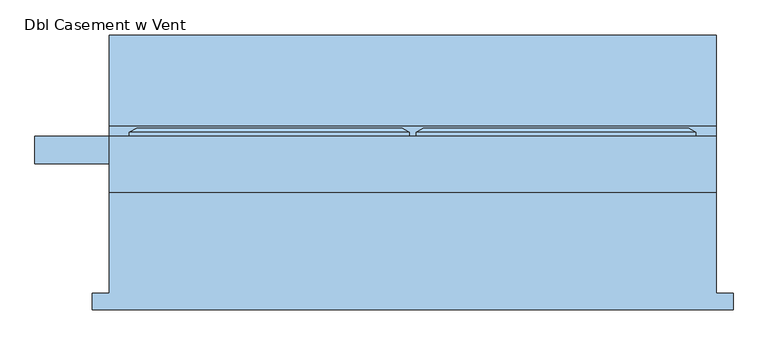
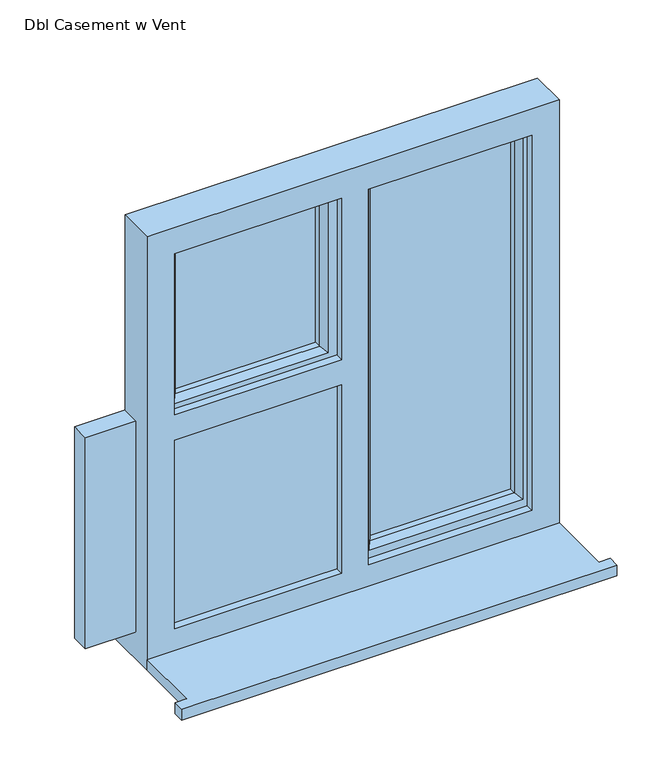
"""IFC4 building model written with IfcOpenShell, lengths in millimetres: window geometry, Dbl Casement w Vent : Doublel Casement with Vent 900w x 1000h."""

from ifc_helpers import new_model, si_unit, frame, origin, place, context, project, spatial, polyline, outline, extrude, faceted_brep, source, transform, mapped, element, save


def dbl_casement_w_vent_ca28e73d(model_context):
    return source(origin(), model_context, "Body", "SolidModel", [
        extrude(outline(polyline([(-760.0, -182.7934322), (-760.0, -157.7934322), (-735.0, -157.7934322), (-735.0, -8.2934322), (165.0, -8.2934322), (165.0, -157.7934322), (190.0, -157.7934322), (190.0, -182.7934322), (-760.0, -182.7934322)])), frame((0.0, 0.0, 1110.0), z_axis=(0.0, 0.0, 1.0), x_axis=(1.0, 0.0, 0.0)), (0.0, 0.0, 1.0), 25.0),
        faceted_brep([(-705.0, 74.7065678, 2080.0), (-705.0, 80.4800705, 2080.0), (-705.0, 80.4800705, 1650.0), (-705.0, 74.7065678, 1650.0), (-695.0, 9.7065678, 2070.0), (-695.0, 74.7065678, 2070.0), (-695.0, 74.7065678, 1660.0), (-695.0, 9.7065678, 1660.0), (-655.0, 24.1994677, 2030.0), (-665.1480377, 9.7065678, 2040.1480377), (-665.1480377, 9.7065678, 1689.8519623), (-655.0, 24.1994677, 1700.0), (-655.0, 38.7065678, 2030.0), (-655.0, 38.7065678, 1700.0), (-665.0, 62.7065678, 2040.0), (-665.0, 38.7065678, 2040.0), (-665.0, 38.7065678, 1690.0), (-665.0, 62.7065678, 1690.0), (-655.0, 80.4800705, 2030.0), (-655.0, 62.7065678, 2030.0), (-655.0, 62.7065678, 1700.0), (-655.0, 80.4800705, 1700.0), (-672.4457548, 86.2535732, 2047.4457548), (-672.4457548, 86.2535732, 1682.5542452), (-694.2153903, 86.2535732, 2069.2153903), (-694.2153903, 86.2535732, 1660.7846097), (-290.0, 80.4800705, 1650.0), (-290.0, 74.7065678, 1650.0), (-300.0, 74.7065678, 1660.0), (-300.0, 9.7065678, 1660.0), (-329.8519623, 9.7065678, 1689.8519623), (-340.0, 24.1994677, 1700.0), (-340.0, 38.7065678, 1700.0), (-330.0, 38.7065678, 1690.0), (-330.0, 62.7065678, 1690.0), (-340.0, 62.7065678, 1700.0), (-340.0, 80.4800705, 1700.0), (-322.5542452, 86.2535732, 1682.5542452), (-300.7846097, 86.2535732, 1660.7846097), (-290.0, 80.4800705, 2080.0), (-290.0, 74.7065678, 2080.0), (-300.0, 74.7065678, 2070.0), (-300.0, 9.7065678, 2070.0), (-329.8519623, 9.7065678, 2040.1480377), (-340.0, 24.1994677, 2030.0), (-340.0, 38.7065678, 2030.0), (-330.0, 38.7065678, 2040.0), (-330.0, 62.7065678, 2040.0), (-340.0, 62.7065678, 2030.0), (-340.0, 80.4800705, 2030.0), (-322.5542452, 86.2535732, 2047.4457548), (-300.7846097, 86.2535732, 2069.2153903)], [[[0, 1, 2, 3]], [[4, 5, 6, 7]], [[8, 9, 10, 11]], [[12, 8, 11, 13]], [[14, 15, 16, 17]], [[18, 19, 20, 21]], [[22, 18, 21, 23]], [[1, 24, 25, 2]], [[3, 2, 26, 27]], [[7, 6, 28, 29]], [[11, 10, 30, 31]], [[13, 11, 31, 32]], [[17, 16, 33, 34]], [[21, 20, 35, 36]], [[23, 21, 36, 37]], [[2, 25, 38, 26]], [[27, 26, 39, 40]], [[29, 28, 41, 42]], [[31, 30, 43, 44]], [[32, 31, 44, 45]], [[34, 33, 46, 47]], [[36, 35, 48, 49]], [[37, 36, 49, 50]], [[26, 38, 51, 39]], [[40, 39, 1, 0]], [[3, 27, 40, 0], [5, 41, 28, 6]], [[42, 41, 5, 4]], [[7, 29, 42, 4], [9, 43, 30, 10]], [[44, 43, 9, 8]], [[45, 44, 8, 12]], [[15, 46, 33, 16], [13, 32, 45, 12]], [[47, 46, 15, 14]], [[17, 34, 47, 14], [19, 48, 35, 20]], [[49, 48, 19, 18]], [[50, 49, 18, 22]], [[24, 51, 38, 25], [23, 37, 50, 22]], [[39, 51, 24, 1]]]),
        extrude(outline(polyline([(95.0, 38.7065678), (-240.0, 38.7065678), (-240.0, 62.7065678), (95.0, 62.7065678), (95.0, 38.7065678)])), frame((0.0, 0.0, 1203.0), z_axis=(0.0, 0.0, 1.0), x_axis=(1.0, 0.0, 0.0)), (0.0, 0.0, 1.0), 837.0),
        extrude(outline(polyline([(-330.0, 38.7065678), (-665.0, 38.7065678), (-665.0, 62.7065678), (-330.0, 62.7065678), (-330.0, 38.7065678)])), frame((0.0, 0.0, 1690.0), z_axis=(0.0, 0.0, 1.0), x_axis=(1.0, 0.0, 0.0)), (0.0, 0.0, 1.0), 350.0),
        extrude(outline(polyline([(-695.0, 33.7065678), (-300.0, 33.7065678), (-300.0, 9.7065678), (-695.0, 9.7065678), (-695.0, 33.7065678)])), frame((0.0, 0.0, 1173.0), z_axis=(0.0, 0.0, 1.0), x_axis=(1.0, 0.0, 0.0)), (0.0, 0.0, 1.0), 457.0),
        faceted_brep([(165.0, -8.2934322, 2110.0), (-735.0, -8.2934322, 2110.0), (-735.0, -8.2934322, 1110.0), (165.0, -8.2934322, 1110.0), (-675.0, -8.2934322, 1185.0), (-675.0, -8.2934322, 1620.0), (-310.0, -8.2934322, 1620.0), (-310.0, -8.2934322, 1185.0), (-675.0, -8.2934322, 2050.0), (-310.0, -8.2934322, 2050.0), (-310.0, -8.2934322, 1678.0), (-675.0, -8.2934322, 1678.0), (-252.0, -8.2934322, 2050.0), (105.0, -8.2934322, 2050.0), (105.0, -8.2934322, 1185.0), (-252.0, -8.2934322, 1185.0), (-735.0, 74.7065678, 2110.0), (-735.0, 74.7065678, 1161.0), (-735.0, 89.7065678, 1159.68767), (-735.0, 89.7065678, 1154.7449676), (-735.0, 224.7065678, 1143.8088847), (-735.0, 224.7065678, 1110.0), (165.0, 74.7065678, 2110.0), (165.0, 74.7065678, 1161.0), (-310.0, 74.7065678, 1173.0), (-310.0, 74.7065678, 1620.0), (-695.0, 74.7065678, 1620.0), (-695.0, 74.7065678, 1173.0), (-310.0, 74.7065678, 2070.0), (-695.0, 74.7065678, 2070.0), (-695.0, 74.7065678, 1660.0), (-310.0, 74.7065678, 1660.0), (125.0, 74.7065678, 1173.0), (125.0, 74.7065678, 2070.0), (-270.0, 74.7065678, 2070.0), (-270.0, 74.7065678, 1173.0), (-695.0, 9.7065678, 2070.0), (-695.0, 9.7065678, 1660.0), (-695.0, 9.7065678, 1630.0), (-695.0, 9.7065678, 1173.0), (-695.0, 33.7065678, 1620.0), (-695.0, 33.7065678, 1630.0), (-300.0, 9.7065678, 2070.0), (-300.0, 9.7065678, 1660.0), (-310.0, 9.7065678, 2050.0), (-675.0, 9.7065678, 2050.0), (-675.0, 9.7065678, 1678.0), (-310.0, 9.7065678, 1678.0), (-270.0, 9.7065678, 2070.0), (125.0, 9.7065678, 2070.0), (125.0, 9.7065678, 1173.0), (-270.0, 9.7065678, 1173.0), (105.0, 9.7065678, 2050.0), (-252.0, 9.7065678, 2050.0), (-252.0, 9.7065678, 1185.0), (105.0, 9.7065678, 1185.0), (-300.0, 9.7065678, 1173.0), (-300.0, 9.7065678, 1630.0), (-675.0, 9.7065678, 1185.0), (-310.0, 9.7065678, 1185.0), (-310.0, 9.7065678, 1620.0), (-675.0, 9.7065678, 1620.0), (-310.0, 33.7065678, 2070.0), (-300.0, 33.7065678, 2070.0), (165.0, 224.7065678, 1110.0), (165.0, 224.7065678, 1143.8088847), (165.0, 89.7065678, 1154.7449676), (165.0, 89.7065678, 1159.68767), (-300.0, 33.7065678, 1660.0), (-300.0, 33.7065678, 1630.0), (-300.0, 33.7065678, 1173.0), (-310.0, 33.7065678, 1660.0), (-310.0, 33.7065678, 1173.0), (-310.0, 33.7065678, 1620.0)], [[[0, 1, 2, 3], [4, 5, 6, 7], [8, 9, 10, 11], [12, 13, 14, 15]], [[1, 16, 17, 18, 19, 20, 21, 2]], [[16, 22, 23, 17], [24, 25, 26, 27], [28, 29, 30, 31], [32, 33, 34, 35]], [[29, 36, 37, 30]], [[38, 39, 27, 26, 40, 41]], [[36, 42, 43, 37], [44, 45, 46, 47]], [[48, 49, 50, 51], [52, 53, 54, 55]], [[56, 39, 38, 57], [58, 59, 60, 61]], [[45, 8, 11, 46]], [[4, 58, 61, 5]], [[1, 0, 22, 16]], [[36, 29, 28, 62, 63, 42]], [[33, 49, 48, 34]], [[8, 45, 44, 9]], [[52, 13, 12, 53]], [[22, 0, 3, 64, 65, 66, 67, 23]], [[33, 32, 50, 49]], [[13, 52, 55, 14]], [[43, 42, 63, 68]], [[69, 70, 56, 57]], [[63, 62, 71, 68]], [[72, 70, 69, 41, 40, 73]], [[62, 28, 31, 71]], [[24, 72, 73, 25]], [[35, 34, 48, 51]], [[53, 12, 15, 54]], [[9, 44, 47, 10]], [[59, 7, 6, 60]], [[64, 3, 2, 21]], [[65, 64, 21, 20]], [[66, 65, 20, 19]], [[67, 66, 19, 18]], [[23, 67, 18, 17]], [[24, 27, 39, 56, 70, 72]], [[32, 35, 51, 50]], [[15, 14, 55, 54]], [[59, 58, 4, 7]], [[57, 38, 41, 69]], [[26, 25, 73, 40]], [[31, 30, 37, 43, 68, 71]], [[47, 46, 11, 10]], [[61, 60, 6, 5]]]),
        extrude(outline(polyline([(1660.0, -675.0), (1660.0, -845.0), (1173.0, -845.0), (1173.0, -310.0), (1343.0, -310.0), (1343.0, -675.0), (1660.0, -675.0)])), frame((0.0, 33.7065678, 0.0), z_axis=(0.0, 1.0, 0.0), x_axis=(0.0, 0.0, 1.0)), (0.0, 0.0, 1.0), 41.0),
        faceted_brep([(-280.0, 74.7065678, 2080.0), (-280.0, 80.4800705, 2080.0), (-280.0, 80.4800705, 1163.0), (-280.0, 74.7065678, 1163.0), (-270.0, 9.7065678, 2070.0), (-270.0, 74.7065678, 2070.0), (-270.0, 74.7065678, 1173.0), (-270.0, 9.7065678, 1173.0), (-230.0, 24.1994677, 2030.0), (-240.1480377, 9.7065678, 2040.1480377), (-240.1480377, 9.7065678, 1202.8519623), (-230.0, 24.1994677, 1213.0), (-230.0, 38.7065678, 2030.0), (-230.0, 38.7065678, 1213.0), (-240.0, 62.7065678, 2040.0), (-240.0, 38.7065678, 2040.0), (-240.0, 38.7065678, 1203.0), (-240.0, 62.7065678, 1203.0), (-230.0, 80.4800705, 2030.0), (-230.0, 62.7065678, 2030.0), (-230.0, 62.7065678, 1213.0), (-230.0, 80.4800705, 1213.0), (-247.4457548, 86.2535732, 2047.4457548), (-247.4457548, 86.2535732, 1195.5542452), (-269.2153903, 86.2535732, 2069.2153903), (-269.2153903, 86.2535732, 1173.7846097), (135.0, 80.4800705, 1163.0), (135.0, 74.7065678, 1163.0), (125.0, 74.7065678, 1173.0), (125.0, 9.7065678, 1173.0), (95.1480377, 9.7065678, 1202.8519623), (85.0, 24.1994677, 1213.0), (85.0, 38.7065678, 1213.0), (95.0, 38.7065678, 1203.0), (95.0, 62.7065678, 1203.0), (85.0, 62.7065678, 1213.0), (85.0, 80.4800705, 1213.0), (102.4457548, 86.2535732, 1195.5542452), (124.2153903, 86.2535732, 1173.7846097), (135.0, 80.4800705, 2080.0), (135.0, 74.7065678, 2080.0), (125.0, 74.7065678, 2070.0), (125.0, 9.7065678, 2070.0), (95.1480377, 9.7065678, 2040.1480377), (85.0, 24.1994677, 2030.0), (85.0, 38.7065678, 2030.0), (95.0, 38.7065678, 2040.0), (95.0, 62.7065678, 2040.0), (85.0, 62.7065678, 2030.0), (85.0, 80.4800705, 2030.0), (102.4457548, 86.2535732, 2047.4457548), (124.2153903, 86.2535732, 2069.2153903)], [[[0, 1, 2, 3]], [[4, 5, 6, 7]], [[8, 9, 10, 11]], [[12, 8, 11, 13]], [[14, 15, 16, 17]], [[18, 19, 20, 21]], [[22, 18, 21, 23]], [[1, 24, 25, 2]], [[3, 2, 26, 27]], [[7, 6, 28, 29]], [[11, 10, 30, 31]], [[13, 11, 31, 32]], [[17, 16, 33, 34]], [[21, 20, 35, 36]], [[23, 21, 36, 37]], [[2, 25, 38, 26]], [[27, 26, 39, 40]], [[29, 28, 41, 42]], [[31, 30, 43, 44]], [[32, 31, 44, 45]], [[34, 33, 46, 47]], [[36, 35, 48, 49]], [[37, 36, 49, 50]], [[26, 38, 51, 39]], [[40, 39, 1, 0]], [[3, 27, 40, 0], [5, 41, 28, 6]], [[42, 41, 5, 4]], [[7, 29, 42, 4], [9, 43, 30, 10]], [[44, 43, 9, 8]], [[45, 44, 8, 12]], [[15, 46, 33, 16], [13, 32, 45, 12]], [[47, 46, 15, 14]], [[17, 34, 47, 14], [19, 48, 35, 20]], [[49, 48, 19, 18]], [[50, 49, 18, 22]], [[24, 51, 38, 25], [23, 37, 50, 22]], [[39, 51, 24, 1]]]),
    ])


if __name__ == "__main__":
    model = new_model("IFC4")
    model_context = context("Model", 3, world=origin())
    ifc_project = project(units=[si_unit("LENGTHUNIT", "METRE", prefix="MILLI")], contexts=[model_context])
    site = spatial("IfcSite", under=ifc_project)
    building = spatial("IfcBuilding", under=site)
    placement = place(None, origin())
    dbl_casement_w_vent_shape = dbl_casement_w_vent_ca28e73d(model_context)
    element("IfcWindow", 1, ObjectType="Dbl Casement w Vent : Doublel Casement with Vent 900w x 1000h", at=placement, inside=building, context=model_context, shape_type="MappedRepresentation", body=[
        mapped(dbl_casement_w_vent_shape, transform((0.0, 0.0, 0.0), x_axis=(1.0, 0.0, 0.0), y_axis=(0.0, 1.0, 0.0), z_axis=(0.0, 0.0, 1.0))),
    ])
    save(model, "model.ifc")

# Revit data of these elements
# Type "Dbl Casement w Vent : Doublel Casement with Vent 900w x 1000h"
#   Type Mark = "73"
#   Operation = "TriplePanelRight"
#   Construction Type Id = "GSP4R"
#   Manufacturer = "Revit"
#   Keynote = "L10"
#   Analytic Construction = "1/8 in Pilkington single glazing"
#   Wrap Layers (Ext) from Ext = 102.5 mm
#   Wrap Layers (Int) from Ext = 177.5 mm
#   Window Board Projection = 25 mm
#   Window Board Extension = 25 mm
#   Visual Light Transmittance = 0.9
#   Vent Depth = 450 mm
#   Thermal Resistance (R) = 0.271106 (m²·K)/W
#   Solar Heat Gain Coefficient = 0.78
#   Rough Width = 900 mm
#   Rough Height = 1000 mm
#   Frame Height = 1350 mm
#   Height = 1000 mm
#   Width = 900 mm
#   Heat Transfer Coefficient (U) = 3.6886 W/(m²·K)
#   Glazing Thickness = 24 mm
#   FrameOffset - External = 100 mm
#   Frame Depth = 65 mm
#   Default Head Height = 2110 mm
#   Cill Depth = 150 mm
#   Cavity Closer Width = 75 mm
#   Cavity Closer Offset from Ext = 110 mm
#   Cavity Closer Depth = 105 mm
#   Vis - Cavity Closers = yes
#   Material Trim = Window Frame
#   Material Glass = Glass
#   Material Frame = Window Frame
#   Wall Closure = (empty or 0)
# Element 1 (IfcWindow, "Dbl Casement w Vent : Doublel Casement with Vent 900w x 1000h")
#   Materials on its faces: "Window Frame", "Glass"
# Materials
#   "Window Frame": class "Miscellaneous", colour RGB 249 249 249, transparency 0, Keynote = "L10"
#   "Glass": class "Glass", colour RGB 0 128 192, transparency 0.9, Description = "Soda Lime Glass", Cost = 0
